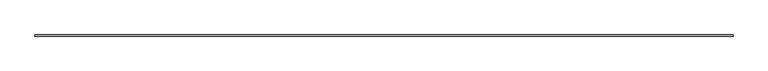
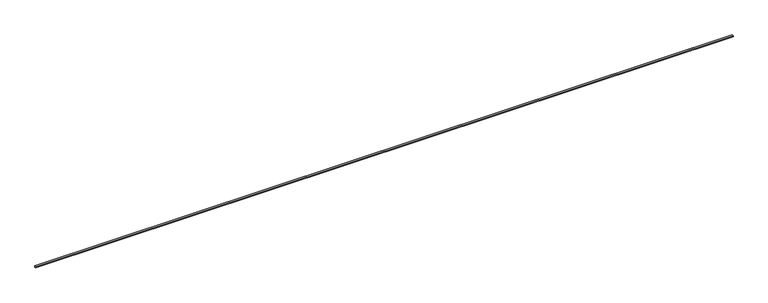
"""IFC4 building model written with IfcOpenShell, lengths in millimetres: proxy geometry, Joint005 3038 : Joint005 3038."""

from ifc_helpers import new_model, si_unit, point, frame, frame_2d, origin, place, context, project, spatial, polyline, circle_curve, trimmed, segment, composite_curve, outline, extrude, source, transform, mapped, element, save


def generic_models_c5dfff9d(model_context):
    return source(origin(), model_context, "Body", "SweptSolid", [
        extrude(outline(composite_curve([segment(polyline([(10407.9541245, 42891.9101563), (10407.9541245, 42887.9921875)]), True, "CONTINUOUS"), segment(trimmed(circle_curve(frame_2d((10406.3557925, 42882.8203125)), 5.4132205), [point((10407.9541245, 42887.9921875))], [point((10404.7574604, 42887.9921875))], True, "CARTESIAN"), True, "CONTINUOUS"), segment(polyline([(10404.7574604, 42887.9921875), (10404.7574604, 42891.9101563)]), True, "CONTINUOUS"), segment(trimmed(circle_curve(frame_2d((10406.3557925, 42886.7382813)), 5.4132205), [point((10404.7574604, 42891.9101563))], [point((10407.9541245, 42891.9101563))], False, "CARTESIAN"), True, "CONTINUOUS")], self_intersect=False)), frame((3694.2883192, 0.0, 0.0), z_axis=(1.0, 0.0, 0.0), x_axis=(0.0, 1.0, 0.0)), (0.0, 0.0, 1.0), 2000.0),
    ])


if __name__ == "__main__":
    model = new_model("IFC4")
    model_context = context("Model", 3, world=origin())
    ifc_project = project(units=[si_unit("LENGTHUNIT", "METRE", prefix="MILLI")], contexts=[model_context])
    site = spatial("IfcSite", under=ifc_project)
    building = spatial("IfcBuilding", under=site)
    placement = place(None, origin())
    generic_models_shape = generic_models_c5dfff9d(model_context)
    element("IfcBuildingElementProxy", 1, Name="Joint005 3038 : Joint005 3038", ObjectType="Joint005 3038 : Joint005 3038", at=placement, inside=building, context=model_context, shape_type="MappedRepresentation", body=[
        mapped(generic_models_shape, transform((0.0, 0.0, 0.0), x_axis=(1.0, 0.0, 0.0), y_axis=(0.0, 1.0, 0.0), z_axis=(0.0, 0.0, 1.0))),
    ])
    save(model, "model.ifc")

# Revit data of these elements
# Type "Joint005 3038 : Joint005 3038"
#   NameOverride = "Joint005"
# Element 1 (IfcBuildingElementProxy, "Joint005 3038 : Joint005 3038")
#   Materials on its faces: "SILICON JOINT"
# Materials
#   "SILICON JOINT": class "Unassigned", colour RGB 150 184 127, transparency 0
